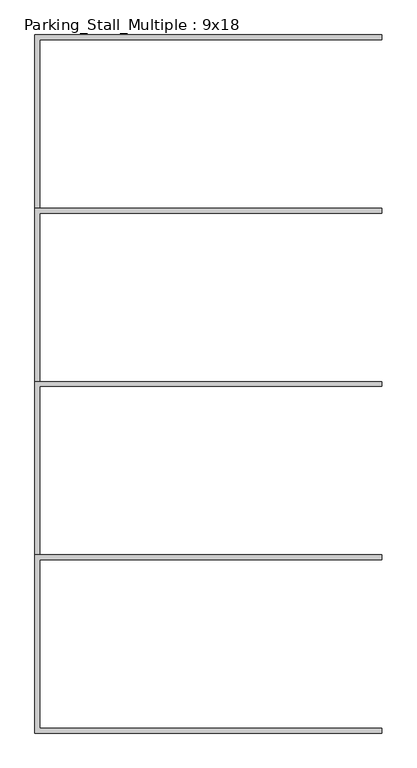
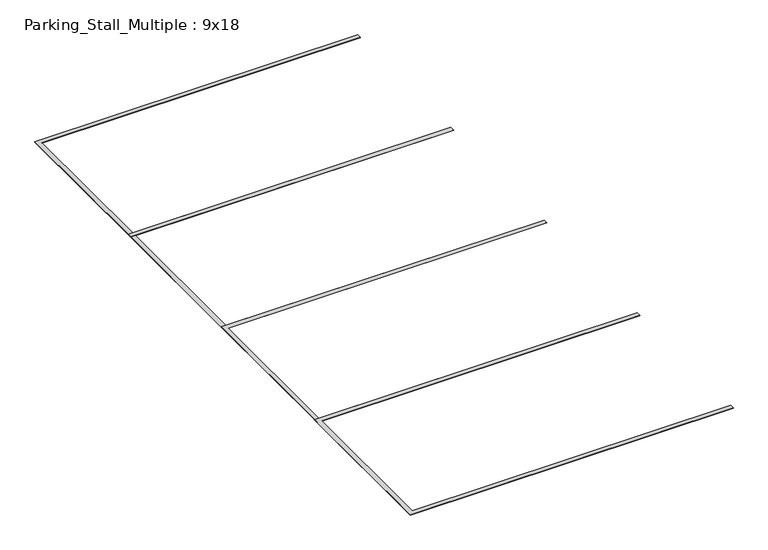
"""IFC4 building model written with IfcOpenShell, lengths in millimetres: proxy geometry, Parking_Stall_Multiple : 9x18."""

from ifc_helpers import new_model, si_unit, origin, origin_with_axes, place, context, project, spatial, polyline, outline, extrude, source, transform, mapped, element, save


def parking_stall_multiple_9x18_c96fd294(model_context):
    return source(origin(), model_context, "Body", "SweptSolid", [
        extrude(outline(polyline([(5486.4, -8229.6), (5486.4, -8305.8), (76.2, -8305.8), (76.2, -10972.8), (5486.4, -10972.8), (5486.4, -11049.0), (0.0, -11049.0), (0.0, -8229.6), (5486.4, -8229.6)])), origin_with_axes(), (0.0, 0.0, 1.0), 6.35),
        extrude(outline(polyline([(5486.4, -5486.4), (5486.4, -5562.6), (76.2, -5562.6), (76.2, -8229.6), (5486.4, -8229.6), (5486.4, -8305.8), (0.0, -8305.8), (0.0, -5486.4), (5486.4, -5486.4)])), origin_with_axes(), (0.0, 0.0, 1.0), 6.35),
        extrude(outline(polyline([(5486.4, -2743.2), (5486.4, -2819.4), (76.2, -2819.4), (76.2, -5486.4), (5486.4, -5486.4), (5486.4, -5562.6), (0.0, -5562.6), (0.0, -2743.2), (5486.4, -2743.2)])), origin_with_axes(), (0.0, 0.0, 1.0), 6.35),
        extrude(outline(polyline([(5486.4, 0.0), (5486.4, -76.2), (76.2, -76.2), (76.2, -2743.2), (5486.4, -2743.2), (5486.4, -2819.4), (0.0, -2819.4), (0.0, 0.0), (5486.4, 0.0)])), origin_with_axes(), (0.0, 0.0, 1.0), 6.35),
    ])


if __name__ == "__main__":
    model = new_model("IFC4")
    model_context = context("Model", 3, world=origin())
    ifc_project = project(units=[si_unit("LENGTHUNIT", "METRE", prefix="MILLI")], contexts=[model_context])
    site = spatial("IfcSite", under=ifc_project)
    building = spatial("IfcBuilding", under=site)
    placement = place(None, origin())
    parking_stall_multiple_9x18_shape = parking_stall_multiple_9x18_c96fd294(model_context)
    element("IfcBuildingElementProxy", 1, Name="Parking_Stall_Multiple : 9x18", ObjectType="Parking_Stall_Multiple : 9x18", at=placement, inside=building, context=model_context, shape_type="MappedRepresentation", body=[
        mapped(parking_stall_multiple_9x18_shape, transform((0.0, 0.0, 0.0), x_axis=(1.0, 0.0, 0.0), y_axis=(0.0, 1.0, 0.0), z_axis=(0.0, 0.0, 1.0))),
    ])
    save(model, "model.ifc")

# Revit data of these elements
# Type "Parking_Stall_Multiple : 9x18"
#   Type Mark = "PK-1"
#   Parking_Width_M = 9' - 0"
#   Parking_Run_Length [instance default] = 65' - 0"
#   Parking_Line_Width = 0' - 3"
#   Parking_Length_M = 18' - 0"
#   Single_Parking_Visibility [instance default] = no
#   Parking_ADA_Symbol = no
#   ParkingUnitsArray [instance default] = 7
#   ParkingUnits [instance default] = 7
#   Multiple_Parking_Visibility [instance default] = yes
#   Parking_Line_Material = none
# Element 1 (IfcBuildingElementProxy, "Parking_Stall_Multiple : 9x18")
#   Parking_Run_Length = 38' - 3.87897"
#   ParkingUnitsArray = 4
#   ParkingUnits = 4
